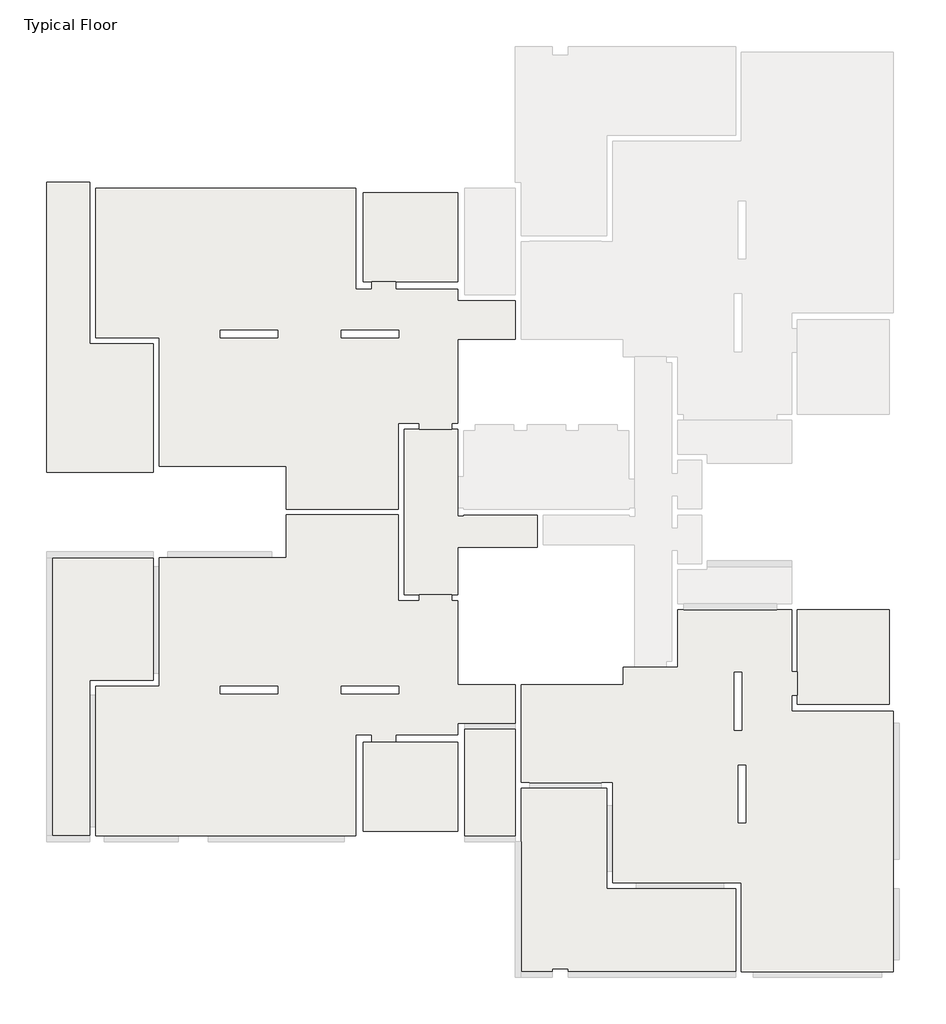
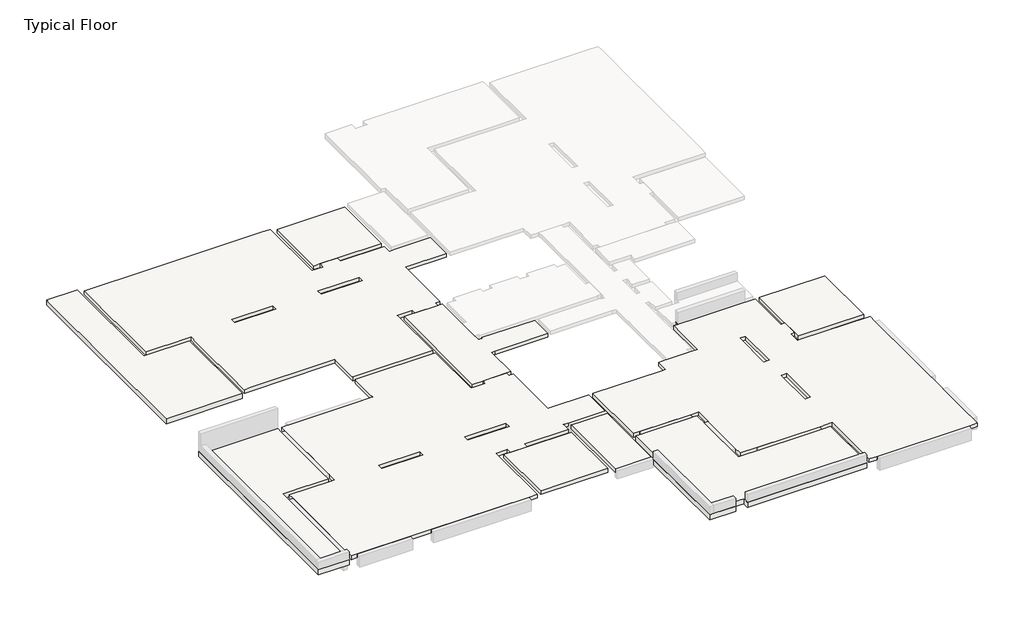
# One storey, part 1 of 2: 11 slabs.
"""IFC4 building model written with IfcOpenShell, lengths in millimetres."""

from ifc_helpers import new_model, si_unit, frame, origin, place, context, project, spatial, polyline, outline, extrude, faceted_brep, element, save

model = new_model("IFC4")

# Units and contexts
model_context = context("Model", 3, world=origin())
ifc_project = project(units=[si_unit("LENGTHUNIT", "METRE", prefix="MILLI")], contexts=[model_context])

# Site, building, storey
site = spatial("IfcSite", under=ifc_project)
building = spatial("IfcBuilding", under=site)
storey = spatial("IfcBuildingStorey", under=building, Name="Typical Floor", Elevation=3000.0)

# Slabs
placement = place(None, origin())
element("IfcSlab", 1, ObjectType="18", at=placement, inside=storey, context=model_context, shape_type="Brep", body=[
    faceted_brep([(-3147.0483227, 11035.7061689, 2820.0), (-2602.0483227, 11035.7061689, 2820.0), (-2602.0483227, 11285.7061689, 2820.0), (-1797.0483227, 11285.7061689, 2820.0), (-1797.0483227, 11035.7061689, 2820.0), (292.9516773, 11035.7061689, 2820.0), (292.9516773, 10641.3507002, 2820.0), (2246.4257984, 10641.3507002, 2820.0), (2246.4257984, 9337.0757978, 2820.0), (306.4257984, 9337.0757978, 2820.0), (306.4257984, 9137.0757978, 2820.0), (306.4257984, 6491.5264814, 2820.0), (96.4257984, 6491.5264814, 2820.0), (96.4257984, 6291.5264814, 2820.0), (-1004.8486157, 6291.5264814, 2820.0), (-1004.8486157, 6491.5264814, 2820.0), (-1704.8486157, 6491.5264814, 2820.0), (-1704.8486157, 6291.5264814, 2820.0), (-1704.8486157, 3590.0103681, 2820.0), (-5499.4457837, 3590.0103681, 2820.0), (-5499.4457837, 3661.3116377, 2820.0), (-5499.4457837, 4839.8443525, 2820.0), (-5499.4457837, 5039.8443525, 2820.0), (-5999.4457837, 5039.8443525, 2820.0), (-9505.5395337, 5039.8443525, 2820.0), (-9805.5395337, 5039.8443525, 2820.0), (-9805.5395337, 5339.8443525, 2820.0), (-9805.5395337, 8939.7491377, 2820.0), (-9805.5395337, 9386.8536298, 2820.0), (-10005.5395337, 9386.8536298, 2820.0), (-11954.2455884, 9386.8536298, 2820.0), (-11954.2455884, 14141.4166181, 2820.0), (-11954.2455884, 14441.4166181, 2820.0), (-11654.2455884, 14441.4166181, 2820.0), (-3147.0483227, 14441.4166181, 2820.0), (-3147.0483227, 11285.7061689, 2820.0), (-5784.0917798, 9641.1944502, 2820.0), (-7730.9496899, 9641.1944502, 2820.0), (-7730.9496899, 9391.1944502, 2820.0), (-5784.0917798, 9391.1944502, 2820.0), (-1703.720686, 9641.1944502, 2820.0), (-3648.408186, 9641.1944502, 2820.0), (-3648.408186, 9391.1944502, 2820.0), (-1703.720686, 9391.1944502, 2820.0), (-2602.0483227, 11035.7061689, 3000.0), (-3147.0483227, 11035.7061689, 3000.0), (-3147.0483227, 11285.7061689, 3000.0), (-3147.0483227, 14441.4166181, 3000.0), (-3547.0483227, 14441.4166181, 3000.0), (-8149.7387524, 14441.4166181, 3000.0), (-9154.7387524, 14441.4166181, 3000.0), (-11654.2455884, 14441.4166181, 3000.0), (-11954.2455884, 14441.4166181, 3000.0), (-11954.2455884, 14141.4166181, 3000.0), (-11954.2455884, 9686.3702314, 3000.0), (-11954.2455884, 9386.8536298, 3000.0), (-10005.5395337, 9386.8536298, 3000.0), (-9805.5395337, 9386.8536298, 3000.0), (-9805.5395337, 8939.7491377, 3000.0), (-9805.5395337, 5339.8443525, 3000.0), (-9805.5395337, 5039.8443525, 3000.0), (-9505.5395337, 5039.8443525, 3000.0), (-5999.4457837, 5039.8443525, 3000.0), (-5499.4457837, 5039.8443525, 3000.0), (-5499.4457837, 4839.8443525, 3000.0), (-5499.4457837, 3661.3116377, 3000.0), (-5499.4457837, 3590.0103681, 3000.0), (-5004.9145337, 3590.0103681, 3000.0), (-1704.8486157, 3590.0103681, 3000.0), (-1704.8486157, 6291.5264814, 3000.0), (-1704.8486157, 6491.5264814, 3000.0), (-1004.8486157, 6491.5264814, 3000.0), (-1004.8486157, 6291.5264814, 3000.0), (96.4257984, 6291.5264814, 3000.0), (96.4257984, 6491.5264814, 3000.0), (306.4257984, 6491.5264814, 3000.0), (306.4257984, 9137.0757978, 3000.0), (306.4257984, 9337.0757978, 3000.0), (2246.4257984, 9337.0757978, 3000.0), (2246.4257984, 10641.3507002, 3000.0), (542.9516773, 10641.3507002, 3000.0), (292.9516773, 10641.3507002, 3000.0), (292.9516773, 11035.7061689, 3000.0), (-1797.0483227, 11035.7061689, 3000.0), (-1797.0483227, 11285.7061689, 3000.0), (-2602.0483227, 11285.7061689, 3000.0), (-7730.9496899, 9641.1944502, 3000.0), (-5784.0917798, 9641.1944502, 3000.0), (-5784.0917798, 9391.1944502, 3000.0), (-7730.9496899, 9391.1944502, 3000.0), (-3648.408186, 9641.1944502, 3000.0), (-1703.720686, 9641.1944502, 3000.0), (-1703.720686, 9391.1944502, 3000.0), (-3648.408186, 9391.1944502, 3000.0)], [[[0, 1, 2, 3, 4, 5, 6, 7, 8, 9, 10, 11, 12, 13, 14, 15, 16, 17, 18, 19, 20, 21, 22, 23, 24, 25, 26, 27, 28, 29, 30, 31, 32, 33, 34, 35], [36, 37, 38, 39], [40, 41, 42, 43]], [[44, 45, 46, 47, 48, 49, 50, 51, 52, 53, 54, 55, 56, 57, 58, 59, 60, 61, 62, 63, 64, 65, 66, 67, 68, 69, 70, 71, 72, 73, 74, 75, 76, 77, 78, 79, 80, 81, 82, 83, 84, 85], [86, 87, 88, 89], [90, 91, 92, 93]], [[45, 0, 35, 34, 47, 46]], [[1, 0, 45, 44]], [[2, 1, 44, 85]], [[3, 2, 85, 84]], [[4, 3, 84, 83]], [[4, 83, 82, 5]], [[79, 7, 6, 81, 80]], [[8, 7, 79, 78]], [[9, 8, 78, 77]], [[9, 77, 76, 75, 11, 10]], [[12, 11, 75, 74]], [[13, 12, 74, 73]], [[14, 13, 73, 72]], [[15, 14, 72, 71]], [[16, 15, 71, 70]], [[16, 70, 69, 68, 18, 17]], [[19, 18, 68, 67, 66]], [[19, 66, 65, 64, 63, 22, 21, 20]], [[22, 63, 62, 61, 60, 25, 24, 23]], [[25, 60, 59, 58, 57, 28, 27, 26]], [[28, 57, 56, 55, 30, 29]], [[30, 55, 54, 53, 52, 32, 31]], [[32, 52, 51, 50, 49, 48, 47, 34, 33]], [[37, 36, 87, 86]], [[38, 37, 86, 89]], [[39, 38, 89, 88]], [[36, 39, 88, 87]], [[41, 40, 91, 90]], [[42, 41, 90, 93]], [[43, 42, 93, 92]], [[40, 43, 92, 91]], [[81, 6, 5, 82]]]),
])
element("IfcSlab", 2, ObjectType="18", at=placement, inside=storey, context=model_context, shape_type="Brep", body=[
    faceted_brep([(292.9516773, 14291.4166181, 2820.0), (292.9516773, 11285.7061689, 2820.0), (-1797.0483227, 11285.7061689, 2820.0), (-2602.0483227, 11285.7061689, 2820.0), (-2897.0483227, 11285.7061689, 2820.0), (-2897.0483227, 14291.4166181, 2820.0), (292.9516773, 11285.7061689, 3000.0), (292.9516773, 14291.4166181, 3000.0), (-2897.0483227, 14291.4166181, 3000.0), (-2897.0483227, 11285.7061689, 3000.0), (-2602.0483227, 11285.7061689, 3000.0), (-1797.0483227, 11285.7061689, 3000.0)], [[[0, 1, 2, 3, 4, 5]], [[6, 7, 8, 9, 10, 11]], [[1, 0, 7, 6]], [[1, 6, 11, 10, 9, 4, 3, 2]], [[5, 4, 9, 8]], [[0, 5, 8, 7]]]),
])
element("IfcSlab", 3, ObjectType="18", at=placement, inside=storey, context=model_context, shape_type="Brep", body=[
    faceted_brep([(-2602.0483227, -4055.6854327, 2820.0), (-3147.0483227, -4055.6854327, 2820.0), (-3147.0483227, -4305.6854327, 2820.0), (-3147.0483227, -7461.3958819, 2820.0), (-3547.0483227, -7461.3958819, 2820.0), (-3547.0483227, -7466.3958819, 2820.0), (-8149.7387524, -7466.3958819, 2820.0), (-8149.7387524, -7461.3958819, 2820.0), (-9154.7387524, -7461.3958819, 2820.0), (-9154.7387524, -7466.3958819, 2820.0), (-11654.2455884, -7466.3958819, 2820.0), (-11654.2455884, -7461.3958819, 2820.0), (-11954.2455884, -7461.3958819, 2820.0), (-11954.2455884, -7161.3958819, 2820.0), (-11954.2455884, -2406.8328936, 2820.0), (-10005.5395337, -2406.8328936, 2820.0), (-9805.5395337, -2406.8328936, 2820.0), (-9805.5395337, -1959.7284014, 2820.0), (-9805.5395337, 1640.1763837, 2820.0), (-9805.5395337, 1940.1763837, 2820.0), (-9505.5395337, 1940.1763837, 2820.0), (-5999.4457837, 1940.1763837, 2820.0), (-5499.4457837, 1940.1763837, 2820.0), (-5499.4457837, 2140.1763837, 2820.0), (-5499.4457837, 3320.5572431, 2820.0), (-5499.4457837, 3390.0103681, 2820.0), (-1704.8486157, 3390.0103681, 2820.0), (-1704.8486157, 491.1895673, 2820.0), (-999.8486157, 491.1895673, 2820.0), (-999.8486157, 688.4942548, 2820.0), (96.4257984, 688.4942548, 2820.0), (96.4257984, 488.4942548, 2820.0), (306.4257984, 488.4942548, 2820.0), (306.4257984, -2157.0550616, 2820.0), (306.4257984, -2357.0550616, 2820.0), (2246.4257984, -2357.0550616, 2820.0), (2246.4257984, -3661.3299639, 2820.0), (292.9516773, -3661.3299639, 2820.0), (292.9516773, -4055.6854327, 2820.0), (-1797.0483227, -4055.6854327, 2820.0), (-1797.0483227, -4305.6854327, 2820.0), (-2602.0483227, -4305.6854327, 2820.0), (-7730.9496899, -2661.1737139, 2820.0), (-5784.0917798, -2661.1737139, 2820.0), (-5784.0917798, -2411.1737139, 2820.0), (-7730.9496899, -2411.1737139, 2820.0), (-3648.408186, -2661.1737139, 2820.0), (-1703.720686, -2661.1737139, 2820.0), (-1703.720686, -2411.1737139, 2820.0), (-3648.408186, -2411.1737139, 2820.0), (-3147.0483227, -4055.6854327, 3000.0), (-2602.0483227, -4055.6854327, 3000.0), (-2602.0483227, -4305.6854327, 3000.0), (-1797.0483227, -4305.6854327, 3000.0), (-1797.0483227, -4055.6854327, 3000.0), (292.9516773, -4055.6854327, 3000.0), (292.9516773, -3661.3299639, 3000.0), (542.9516773, -3661.3299639, 3000.0), (2246.4257984, -3661.3299639, 3000.0), (2246.4257984, -2357.0550616, 3000.0), (306.4257984, -2357.0550616, 3000.0), (306.4257984, -2157.0550616, 3000.0), (306.4257984, 488.4942548, 3000.0), (96.4257984, 488.4942548, 3000.0), (96.4257984, 688.4942548, 3000.0), (-999.8486157, 688.4942548, 3000.0), (-999.8486157, 491.1895673, 3000.0), (-1504.8486157, 491.1895673, 3000.0), (-1704.8486157, 491.1895673, 3000.0), (-1704.8486157, 3390.0103681, 3000.0), (-5004.9145337, 3390.0103681, 3000.0), (-5499.4457837, 3390.0103681, 3000.0), (-5499.4457837, 3320.5572431, 3000.0), (-5499.4457837, 2140.1763837, 3000.0), (-5499.4457837, 1940.1763837, 3000.0), (-5999.4457837, 1940.1763837, 3000.0), (-9505.5395337, 1940.1763837, 3000.0), (-9805.5395337, 1940.1763837, 3000.0), (-9805.5395337, 1640.1763837, 3000.0), (-9805.5395337, -1959.7284014, 3000.0), (-9805.5395337, -2406.8328936, 3000.0), (-10005.5395337, -2406.8328936, 3000.0), (-11954.2455884, -2406.8328936, 3000.0), (-11954.2455884, -2706.3494952, 3000.0), (-11954.2455884, -7161.3958819, 3000.0), (-11954.2455884, -7461.3958819, 3000.0), (-11654.2455884, -7461.3958819, 3000.0), (-11654.2455884, -7466.3958819, 3000.0), (-9154.7387524, -7466.3958819, 3000.0), (-9154.7387524, -7461.3958819, 3000.0), (-8149.7387524, -7461.3958819, 3000.0), (-8149.7387524, -7466.3958819, 3000.0), (-3547.0483227, -7466.3958819, 3000.0), (-3547.0483227, -7461.3958819, 3000.0), (-3147.0483227, -7461.3958819, 3000.0), (-3147.0483227, -4305.6854327, 3000.0), (-5784.0917798, -2661.1737139, 3000.0), (-7730.9496899, -2661.1737139, 3000.0), (-7730.9496899, -2411.1737139, 3000.0), (-5784.0917798, -2411.1737139, 3000.0), (-1703.720686, -2661.1737139, 3000.0), (-3648.408186, -2661.1737139, 3000.0), (-3648.408186, -2411.1737139, 3000.0), (-1703.720686, -2411.1737139, 3000.0)], [[[0, 1, 2, 3, 4, 5, 6, 7, 8, 9, 10, 11, 12, 13, 14, 15, 16, 17, 18, 19, 20, 21, 22, 23, 24, 25, 26, 27, 28, 29, 30, 31, 32, 33, 34, 35, 36, 37, 38, 39, 40, 41], [42, 43, 44, 45], [46, 47, 48, 49]], [[50, 51, 52, 53, 54, 55, 56, 57, 58, 59, 60, 61, 62, 63, 64, 65, 66, 67, 68, 69, 70, 71, 72, 73, 74, 75, 76, 77, 78, 79, 80, 81, 82, 83, 84, 85, 86, 87, 88, 89, 90, 91, 92, 93, 94, 95], [96, 97, 98, 99], [100, 101, 102, 103]], [[1, 50, 95, 94, 3, 2]], [[1, 0, 51, 50]], [[0, 41, 52, 51]], [[41, 40, 53, 52]], [[40, 39, 54, 53]], [[54, 39, 38, 55]], [[36, 58, 57, 56, 37]], [[36, 35, 59, 58]], [[35, 34, 60, 59]], [[32, 62, 61, 60, 34, 33]], [[32, 31, 63, 62]], [[31, 30, 64, 63]], [[64, 30, 29, 65]], [[26, 69, 68, 27]], [[26, 25, 71, 70, 69]], [[22, 74, 73, 72, 71, 25, 24, 23]], [[19, 77, 76, 75, 74, 22, 21, 20]], [[16, 80, 79, 78, 77, 19, 18, 17]], [[14, 82, 81, 80, 16, 15]], [[82, 14, 13, 12, 85, 84, 83]], [[87, 10, 9, 88]], [[91, 6, 5, 92]], [[43, 42, 97, 96]], [[42, 45, 98, 97]], [[45, 44, 99, 98]], [[44, 43, 96, 99]], [[47, 46, 101, 100]], [[46, 49, 102, 101]], [[49, 48, 103, 102]], [[48, 47, 100, 103]], [[86, 11, 10, 87]], [[11, 86, 85, 12]], [[27, 68, 67, 66, 28]], [[28, 66, 65, 29]], [[37, 56, 55, 38]], [[7, 90, 89, 8]], [[90, 7, 6, 91]], [[8, 89, 88, 9]], [[93, 4, 3, 94]], [[4, 93, 92, 5]]]),
])
element("IfcSlab", 4, ObjectType="18", at=placement, inside=storey, context=model_context, shape_type="Brep", body=[
    faceted_brep([(292.9516773, -4305.6854327, 2820.0), (292.9516773, -7311.3958819, 2820.0), (-2897.0483227, -7311.3958819, 2820.0), (-2897.0483227, -4305.6854327, 2820.0), (-2602.0483227, -4305.6854327, 2820.0), (-1797.0483227, -4305.6854327, 2820.0), (292.9516773, -7311.3958819, 3000.0), (292.9516773, -4305.6854327, 3000.0), (-1797.0483227, -4305.6854327, 3000.0), (-2602.0483227, -4305.6854327, 3000.0), (-2897.0483227, -4305.6854327, 3000.0), (-2897.0483227, -7311.3958819, 3000.0)], [[[0, 1, 2, 3, 4, 5]], [[6, 7, 8, 9, 10, 11]], [[1, 0, 7, 6]], [[3, 10, 9, 8, 7, 0, 5, 4]], [[3, 2, 11, 10]], [[2, 1, 6, 11]]]),
])
element("IfcSlab", 5, ObjectType="18", at=placement, inside=storey, context=model_context, shape_type="SweptSolid", body=[
    extrude(outline(polyline([(2246.4257984, -3861.3299639), (2246.4257984, -7461.3958819), (542.9516773, -7461.3958819), (542.9516773, -3861.3299639), (2246.4257984, -3861.3299639)])), frame((0.0, 0.0, 2820.0), z_axis=(0.0, 0.0, 1.0), x_axis=(1.0, 0.0, 0.0)), (0.0, 0.0, 1.0), 180.0),
])
element("IfcSlab", 6, ObjectType="18", at=placement, inside=storey, context=model_context, shape_type="Brep", body=[
    faceted_brep([(11796.5527515, -2710.0457842, 2820.0), (11596.5527515, -2710.0457842, 2820.0), (11596.5527515, -3259.804085, 2820.0), (15047.1826343, -3259.804085, 2820.0), (15047.1826343, -12061.3104327, 2820.0), (14652.4902515, -12061.3104327, 2820.0), (14652.4902515, -12066.3104327, 2820.0), (10302.4292163, -12066.3104327, 2820.0), (10302.4292163, -12061.3104327, 2820.0), (9902.4292163, -12061.3104327, 2820.0), (9902.4292163, -9261.9354327, 2820.0), (9902.4292163, -9061.9354327, 2820.0), (9302.4292163, -9061.9354327, 2820.0), (6350.1123218, -9061.9354327, 2820.0), (5545.4492359, -9061.9354327, 2820.0), (5545.4492359, -8661.9549639, 2820.0), (5545.4492359, -6456.8182452, 2820.0), (5545.4492359, -5860.2777178, 2820.0), (5545.4492359, -5660.2777178, 2820.0), (5152.6049976, -5660.2777178, 2820.0), (5152.6049976, -5665.2777178, 2820.0), (2745.6201343, -5665.2777178, 2820.0), (2745.6201343, -5660.2777178, 2820.0), (2446.4257984, -5660.2777178, 2820.0), (2446.4257984, -2357.0550616, 2820.0), (5901.4257984, -2357.0550616, 2820.0), (5901.4257984, -1759.7284014, 2820.0), (6296.4111499, -1759.7284014, 2820.0), (7351.2304859, -1759.7284014, 2820.0), (7351.2304859, -1760.3729327, 2820.0), (7751.2304859, -1760.3729327, 2820.0), (7751.2304859, -1560.3729327, 2820.0), (7751.2304859, 188.6553877, 2820.0), (7955.5859546, 188.6553877, 2820.0), (7955.5859546, 388.6553877, 2820.0), (11103.869646, 388.6553877, 2820.0), (11103.869646, 188.6553877, 2820.0), (11596.5527515, 188.6553877, 2820.0), (11596.5527515, -1909.8089678, 2820.0), (11796.5527515, -1909.8089678, 2820.0), (10046.8798999, -7025.4657061, 2820.0), (10046.8798999, -5082.9486163, 2820.0), (9796.8798999, -5082.9486163, 2820.0), (9796.8798999, -7025.4657061, 2820.0), (9906.2060718, -3891.3934405, 2820.0), (9906.2060718, -1940.19471, 2820.0), (9656.2060718, -1940.19471, 2820.0), (9656.2060718, -3891.3934405, 2820.0), (11596.5527515, -2710.0457842, 3000.0), (11796.5527515, -2710.0457842, 3000.0), (11796.5527515, -1909.8089678, 3000.0), (11596.5527515, -1909.8089678, 3000.0), (11596.5527515, 188.6553877, 3000.0), (11103.869646, 188.6553877, 3000.0), (11103.869646, 388.6553877, 3000.0), (7955.5859546, 388.6553877, 3000.0), (7955.5859546, 188.6553877, 3000.0), (7751.2304859, 188.6553877, 3000.0), (7751.2304859, -1560.3729327, 3000.0), (7751.2304859, -1760.3729327, 3000.0), (7351.2304859, -1760.3729327, 3000.0), (7351.2304859, -1759.7284014, 3000.0), (6296.4111499, -1759.7284014, 3000.0), (5901.4257984, -1759.7284014, 3000.0), (5901.4257984, -2357.0550616, 3000.0), (5701.4257984, -2357.0550616, 3000.0), (2446.4257984, -2357.0550616, 3000.0), (2446.4257984, -5660.2777178, 3000.0), (2745.6201343, -5660.2777178, 3000.0), (2745.6201343, -5665.2777178, 3000.0), (5152.6049976, -5665.2777178, 3000.0), (5152.6049976, -5660.2777178, 3000.0), (5545.4492359, -5660.2777178, 3000.0), (5545.4492359, -5860.2777178, 3000.0), (5545.4492359, -6456.8182452, 3000.0), (5545.4492359, -8661.9549639, 3000.0), (5545.4492359, -9061.9354327, 3000.0), (6350.1123218, -9061.9354327, 3000.0), (9302.4292163, -9061.9354327, 3000.0), (9902.4292163, -9061.9354327, 3000.0), (9902.4292163, -9261.9354327, 3000.0), (9902.4292163, -12061.3104327, 3000.0), (10302.4292163, -12061.3104327, 3000.0), (10302.4292163, -12066.3104327, 3000.0), (14652.4902515, -12066.3104327, 3000.0), (14652.4902515, -12061.3104327, 3000.0), (15047.1826343, -12061.3104327, 3000.0), (15047.1826343, -11661.3104327, 3000.0), (15047.1826343, -9252.3065264, 3000.0), (15047.1826343, -8260.429085, 3000.0), (15047.1826343, -3654.8187334, 3000.0), (15047.1826343, -3259.804085, 3000.0), (11796.5527515, -3259.804085, 3000.0), (11596.5527515, -3259.804085, 3000.0), (11596.5527515, -2710.6903155, 3000.0), (10046.8798999, -5082.9486163, 3000.0), (10046.8798999, -7025.4657061, 3000.0), (9796.8798999, -7025.4657061, 3000.0), (9796.8798999, -5082.9486163, 3000.0), (9906.2060718, -1940.19471, 3000.0), (9906.2060718, -3891.3934405, 3000.0), (9656.2060718, -3891.3934405, 3000.0), (9656.2060718, -1940.19471, 3000.0)], [[[0, 1, 2, 3, 4, 5, 6, 7, 8, 9, 10, 11, 12, 13, 14, 15, 16, 17, 18, 19, 20, 21, 22, 23, 24, 25, 26, 27, 28, 29, 30, 31, 32, 33, 34, 35, 36, 37, 38, 39], [40, 41, 42, 43], [44, 45, 46, 47]], [[48, 49, 50, 51, 52, 53, 54, 55, 56, 57, 58, 59, 60, 61, 62, 63, 64, 65, 66, 67, 68, 69, 70, 71, 72, 73, 74, 75, 76, 77, 78, 79, 80, 81, 82, 83, 84, 85, 86, 87, 88, 89, 90, 91, 92, 93, 94], [95, 96, 97, 98], [99, 100, 101, 102]], [[69, 21, 20, 70]], [[14, 76, 75, 74, 73, 72, 18, 17, 16, 15]], [[11, 79, 78, 77, 76, 14, 13, 12]], [[79, 11, 10, 9, 81, 80]], [[83, 7, 6, 84]], [[3, 91, 90, 89, 88, 87, 86, 4]], [[1, 48, 94, 93, 2]], [[1, 0, 49, 48]], [[49, 0, 39, 50]], [[51, 38, 37, 52]], [[30, 59, 58, 57, 32, 31]], [[26, 63, 62, 61, 28, 27]], [[63, 26, 25, 64]], [[66, 24, 23, 67]], [[22, 68, 67, 23]], [[68, 22, 21, 69]], [[18, 72, 71, 19]], [[19, 71, 70, 20]], [[40, 96, 95, 41]], [[42, 98, 97, 43]], [[41, 95, 98, 42]], [[96, 40, 43, 97]], [[44, 100, 99, 45]], [[46, 102, 101, 47]], [[45, 99, 102, 46]], [[100, 44, 47, 101]], [[91, 3, 2, 93, 92]], [[38, 51, 50, 39]], [[36, 53, 52, 37]], [[29, 60, 59, 30]], [[60, 29, 28, 61]], [[56, 33, 32, 57]], [[33, 56, 55, 34]], [[35, 34, 55, 54]], [[53, 36, 35, 54]], [[64, 25, 24, 66, 65]], [[8, 82, 81, 9]], [[82, 8, 7, 83]], [[85, 5, 4, 86]], [[5, 85, 84, 6]]]),
])
element("IfcSlab", 7, ObjectType="18", at=placement, inside=storey, context=model_context, shape_type="Brep", body=[
    faceted_brep([(14897.1826343, 188.5748212, 2820.0), (14897.1826343, -3009.804085, 2820.0), (11796.5527515, -3009.804085, 2820.0), (11796.5527515, -2710.0457842, 2820.0), (11796.5527515, -1909.8089678, 2820.0), (11796.5527515, -1909.1644366, 2820.0), (11796.5527515, 188.5748212, 2820.0), (14897.1826343, -3009.804085, 3000.0), (14897.1826343, 188.5748212, 3000.0), (11796.5527515, 188.5748212, 3000.0), (11796.5527515, -1909.1644366, 3000.0), (11796.5527515, -1909.8089678, 3000.0), (11796.5527515, -2710.0457842, 3000.0), (11796.5527515, -2710.6903155, 3000.0), (11796.5527515, -3009.804085, 3000.0)], [[[0, 1, 2, 3, 4, 5, 6]], [[7, 8, 9, 10, 11, 12, 13, 14]], [[1, 0, 8, 7]], [[0, 6, 9, 8]], [[2, 14, 13, 12, 11, 10, 9, 6, 5, 4, 3]], [[2, 1, 7, 14]]]),
])
element("IfcSlab", 8, ObjectType="18", at=placement, inside=storey, context=model_context, shape_type="Brep", body=[
    faceted_brep([(306.4257984, 6291.5264814, 2820.0), (306.4257984, 4687.0757978, 2820.0), (306.4257984, 3635.0909345, 2820.0), (301.7382984, 3635.0909345, 2820.0), (301.7382984, 3340.0909345, 2820.0), (501.7382984, 3340.0909345, 2820.0), (501.7382984, 3385.0909345, 2820.0), (2997.0654468, 3385.0909345, 2820.0), (2997.0654468, 2292.9449384, 2820.0), (506.4257984, 2292.9449384, 2820.0), (306.4257984, 2292.9449384, 2820.0), (306.4257984, 688.4942548, 2820.0), (96.4257984, 688.4942548, 2820.0), (-999.8486157, 688.4942548, 2820.0), (-999.8486157, 691.1895673, 2820.0), (-1504.8486157, 691.1895673, 2820.0), (-1504.8486157, 6291.5264814, 2820.0), (-1004.8486157, 6291.5264814, 2820.0), (96.4257984, 6291.5264814, 2820.0), (306.4257984, 4687.0757978, 3000.0), (306.4257984, 6291.5264814, 3000.0), (96.4257984, 6291.5264814, 3000.0), (-1004.8486157, 6291.5264814, 3000.0), (-1504.8486157, 6291.5264814, 3000.0), (-1504.8486157, 691.1895673, 3000.0), (-999.8486157, 691.1895673, 3000.0), (-999.8486157, 688.4942548, 3000.0), (96.4257984, 688.4942548, 3000.0), (306.4257984, 688.4942548, 3000.0), (306.4257984, 2292.9449384, 3000.0), (506.4257984, 2292.9449384, 3000.0), (2997.0654468, 2292.9449384, 3000.0), (2997.0654468, 3385.0909345, 3000.0), (501.7382984, 3385.0909345, 3000.0), (501.7382984, 3340.0909345, 3000.0), (301.7382984, 3340.0909345, 3000.0), (301.7382984, 3635.0909345, 3000.0), (306.4257984, 3635.0909345, 3000.0)], [[[0, 1, 2, 3, 4, 5, 6, 7, 8, 9, 10, 11, 12, 13, 14, 15, 16, 17, 18]], [[19, 20, 21, 22, 23, 24, 25, 26, 27, 28, 29, 30, 31, 32, 33, 34, 35, 36, 37]], [[1, 0, 20, 19]], [[2, 1, 19, 37]], [[3, 2, 37, 36]], [[4, 3, 36, 35]], [[5, 4, 35, 34]], [[6, 5, 34, 33]], [[7, 6, 33, 32]], [[8, 7, 32, 31]], [[9, 8, 31, 30]], [[10, 9, 30, 29]], [[11, 10, 29, 28]], [[11, 28, 27, 26, 13, 12]], [[14, 13, 26, 25]], [[15, 14, 25, 24]], [[16, 15, 24, 23]], [[16, 23, 22, 21, 20, 0, 18, 17]]]),
])
element("IfcSlab", 9, ObjectType="25", at=placement, inside=storey, context=model_context, shape_type="Brep", body=[
    faceted_brep([(-10005.5395337, 4839.8443525, 2750.0), (-13614.2455884, 4839.8443525, 2750.0), (-13614.2455884, 14641.4166181, 2750.0), (-12154.2455884, 14641.4166181, 2750.0), (-12154.2455884, 14141.4166181, 2750.0), (-12154.2455884, 9686.3702314, 2750.0), (-12154.2455884, 9186.8536298, 2750.0), (-11954.2455884, 9186.8536298, 2750.0), (-10005.5395337, 9186.8536298, 2750.0), (-13614.2455884, 4839.8443525, 3000.0), (-13414.2455884, 4839.8443525, 3000.0), (-10005.5395337, 4839.8443525, 3000.0), (-10005.5395337, 5039.8443525, 3000.0), (-10005.5395337, 5339.8443525, 3000.0), (-10005.5395337, 8939.7491377, 3000.0), (-10005.5395337, 9186.8536298, 3000.0), (-11954.2455884, 9186.8536298, 3000.0), (-12154.2455884, 9186.8536298, 3000.0), (-12154.2455884, 9686.3702314, 3000.0), (-12154.2455884, 14141.4166181, 3000.0), (-12154.2455884, 14441.4166181, 3000.0), (-12154.2455884, 14641.4166181, 3000.0), (-13614.2455884, 14641.4166181, 3000.0), (-13614.2455884, 14441.4166181, 3000.0)], [[[0, 1, 2, 3, 4, 5, 6, 7, 8]], [[9, 10, 11, 12, 13, 14, 15, 16, 17, 18, 19, 20, 21, 22, 23]], [[1, 0, 11, 10, 9]], [[2, 1, 9, 23, 22]], [[3, 2, 22, 21]], [[3, 21, 20, 19, 18, 17, 6, 5, 4]], [[6, 17, 16, 15, 8, 7]], [[0, 8, 15, 14, 13, 12, 11]]]),
])
element("IfcSlab", 10, ObjectType="25", at=placement, inside=storey, context=model_context, shape_type="Brep", body=[
    faceted_brep([(-13614.2455884, 2140.1763837, 2750.0), (-10005.5395337, 2140.1763837, 2750.0), (-10005.5395337, -2206.8328936, 2750.0), (-11954.2455884, -2206.8328936, 2750.0), (-12154.2455884, -2206.8328936, 2750.0), (-12154.2455884, -2706.3494952, 2750.0), (-12154.2455884, -7161.3958819, 2750.0), (-12154.2455884, -7661.3958819, 2750.0), (-13614.2455884, -7661.3958819, 2750.0), (-10005.5395337, 2140.1763837, 3000.0), (-13414.2455884, 2140.1763837, 3000.0), (-13614.2455884, 2140.1763837, 3000.0), (-13614.2455884, -7461.3958819, 3000.0), (-13614.2455884, -7661.3958819, 3000.0), (-12154.2455884, -7661.3958819, 3000.0), (-12154.2455884, -7461.3958819, 3000.0), (-12154.2455884, -7161.3958819, 3000.0), (-12154.2455884, -2706.3494952, 3000.0), (-12154.2455884, -2206.8328936, 3000.0), (-11954.2455884, -2206.8328936, 3000.0), (-10005.5395337, -2206.8328936, 3000.0), (-10005.5395337, -1959.7284014, 3000.0), (-10005.5395337, 1640.1763837, 3000.0), (-10005.5395337, 1940.1763837, 3000.0)], [[[0, 1, 2, 3, 4, 5, 6, 7, 8]], [[9, 10, 11, 12, 13, 14, 15, 16, 17, 18, 19, 20, 21, 22, 23]], [[1, 0, 11, 10, 9]], [[0, 8, 13, 12, 11]], [[8, 7, 14, 13]], [[4, 18, 17, 16, 15, 14, 7, 6, 5]], [[2, 20, 19, 18, 4, 3]], [[2, 1, 9, 23, 22, 21, 20]]]),
])
element("IfcSlab", 11, ObjectType="25", at=placement, inside=storey, context=model_context, shape_type="Brep", body=[
    faceted_brep([(3495.6958179, -12260.9784014, 2750.0), (2246.4257984, -12260.9784014, 2750.0), (2246.4257984, -7661.3958819, 2750.0), (2446.4257984, -7661.3958819, 2750.0), (2446.4257984, -5860.2777178, 2750.0), (5345.4492359, -5860.2777178, 2750.0), (5345.4492359, -6456.8182452, 2750.0), (5345.4492359, -8661.9549639, 2750.0), (5345.4492359, -9261.9354327, 2750.0), (5545.4492359, -9261.9354327, 2750.0), (6350.1123218, -9261.9354327, 2750.0), (9302.4292163, -9261.9354327, 2750.0), (9702.4292163, -9261.9354327, 2750.0), (9702.4292163, -12261.3104327, 2750.0), (4045.6958179, -12261.3104327, 2750.0), (4045.6958179, -12260.9784014, 2750.0), (4045.6958179, -11960.9784014, 2750.0), (3495.6958179, -11960.9784014, 2750.0), (2246.4257984, -12260.9784014, 3000.0), (2446.4257984, -12260.9784014, 3000.0), (3495.6958179, -12260.9784014, 3000.0), (3495.6958179, -12060.9784014, 3000.0), (3495.6958179, -11960.9784014, 3000.0), (4045.6958179, -11960.9784014, 3000.0), (4045.6958179, -12061.3104327, 3000.0), (4045.6958179, -12260.9784014, 3000.0), (4045.6958179, -12261.3104327, 3000.0), (9702.4292163, -12261.3104327, 3000.0), (9702.4292163, -12061.3104327, 3000.0), (9702.4292163, -9261.9354327, 3000.0), (9302.4292163, -9261.9354327, 3000.0), (6350.1123218, -9261.9354327, 3000.0), (5545.4492359, -9261.9354327, 3000.0), (5345.4492359, -9261.9354327, 3000.0), (5345.4492359, -8661.9549639, 3000.0), (5345.4492359, -6456.8182452, 3000.0), (5345.4492359, -5860.2777178, 3000.0), (5152.6049976, -5860.2777178, 3000.0), (2745.6201343, -5860.2777178, 3000.0), (2446.4257984, -5860.2777178, 3000.0), (2446.4257984, -7661.3958819, 3000.0), (2246.4257984, -7661.3958819, 3000.0)], [[[0, 1, 2, 3, 4, 5, 6, 7, 8, 9, 10, 11, 12, 13, 14, 15, 16, 17]], [[18, 19, 20, 21, 22, 23, 24, 25, 26, 27, 28, 29, 30, 31, 32, 33, 34, 35, 36, 37, 38, 39, 40, 41]], [[1, 0, 20, 19, 18]], [[0, 17, 22, 21, 20]], [[17, 16, 23, 22]], [[14, 26, 25, 24, 23, 16, 15]], [[14, 13, 27, 26]], [[13, 12, 29, 28, 27]], [[8, 33, 32, 31, 30, 29, 12, 11, 10, 9]], [[5, 36, 35, 34, 33, 8, 7, 6]], [[5, 4, 39, 38, 37, 36]], [[2, 1, 18, 41]], [[3, 2, 41, 40]], [[4, 3, 40, 39]]]),
])

save(model, "model.ifc")

# Revit data of these elements
# Type "18"
#   Function = 0
#   Layers, outside or top first: 18 cm "Concrete" (function 1)
# Type "25"
#   Function = 0
#   Layers, outside or top first: 25 cm "Concrete" (function 1)
# Element 1 (IfcSlab, "18")
#   Mark = "S5"
#   SOFiSTiK_AMG_Comments = ""
#   Height Offset From Level = 0 cm
#   built-in parameter 1001954 = 1
#   SOFiSTiK_AMG_Scheduled = yes
#   SOFiSTiK_AMG_Adjusted = yes
#   Phase Created = New Construction
#   Materials on its faces: "Concrete"
# Element 2 (IfcSlab, "18")
#   Mark = "S6"
#   SOFiSTiK_AMG_Comments = ""
#   Height Offset From Level = 0 cm
#   built-in parameter 1001954 = 1
#   SOFiSTiK_AMG_Scheduled = yes
#   SOFiSTiK_AMG_Adjusted = yes
#   Phase Created = New Construction
#   Materials on its faces: "Concrete"
# Element 3 (IfcSlab, "18")
#   Mark = "S10"
#   SOFiSTiK_AMG_Comments = ""
#   Height Offset From Level = 0 cm
#   built-in parameter 1001954 = 1
#   SOFiSTiK_AMG_Scheduled = yes
#   SOFiSTiK_AMG_Adjusted = yes
#   Phase Created = New Construction
#   Materials on its faces: "Concrete"
# Element 4 (IfcSlab, "18")
#   Mark = "S11"
#   SOFiSTiK_AMG_Comments = ""
#   Height Offset From Level = 0 cm
#   built-in parameter 1001954 = 1
#   SOFiSTiK_AMG_Scheduled = yes
#   SOFiSTiK_AMG_Adjusted = yes
#   Phase Created = New Construction
#   Materials on its faces: "Concrete"
# Element 5 (IfcSlab, "18")
#   Mark = "S12"
#   SOFiSTiK_AMG_Comments = ""
#   Height Offset From Level = 0 cm
#   built-in parameter 1001954 = 1
#   SOFiSTiK_AMG_Scheduled = yes
#   SOFiSTiK_AMG_Adjusted = yes
#   Phase Created = New Construction
#   Materials on its faces: "Concrete"
# Element 6 (IfcSlab, "18")
#   Mark = "S13"
#   SOFiSTiK_AMG_Comments = ""
#   built-in parameter 1001955 = -1.5708 (stored number, unit not read)
#   Height Offset From Level = 0 cm
#   built-in parameter 1001954 = 1
#   SOFiSTiK_AMG_Scheduled = yes
#   SOFiSTiK_AMG_Adjusted = yes
#   Phase Created = New Construction
#   Materials on its faces: "Concrete"
# Element 7 (IfcSlab, "18")
#   Mark = "S14"
#   SOFiSTiK_AMG_Comments = ""
#   Height Offset From Level = 0 cm
#   built-in parameter 1001954 = 1
#   SOFiSTiK_AMG_Scheduled = yes
#   SOFiSTiK_AMG_Adjusted = yes
#   Phase Created = New Construction
#   Materials on its faces: "Concrete"
# Element 8 (IfcSlab, "18")
#   Mark = "S18"
#   SOFiSTiK_AMG_Comments = ""
#   Height Offset From Level = 0 cm
#   built-in parameter 1001954 = 1
#   SOFiSTiK_AMG_Scheduled = yes
#   SOFiSTiK_AMG_Adjusted = no
#   Phase Created = New Construction
#   Materials on its faces: "Concrete"
# Element 9 (IfcSlab, "25")
#   Mark = "S1"
#   SOFiSTiK_AMG_Comments = ""
#   Height Offset From Level = 0 cm
#   built-in parameter 1001954 = 1
#   SOFiSTiK_AMG_Scheduled = yes
#   SOFiSTiK_AMG_Adjusted = yes
#   Phase Created = New Construction
#   Materials on its faces: "Concrete"
# Element 10 (IfcSlab, "25")
#   Mark = "S3"
#   SOFiSTiK_AMG_Comments = ""
#   Height Offset From Level = 0 cm
#   built-in parameter 1001954 = 1
#   SOFiSTiK_AMG_Scheduled = yes
#   SOFiSTiK_AMG_Adjusted = yes
#   Phase Created = New Construction
#   Materials on its faces: "Concrete"
# Element 11 (IfcSlab, "25")
#   Mark = "S4"
#   SOFiSTiK_AMG_Comments = ""
#   built-in parameter 1001955 = -1.5708 (stored number, unit not read)
#   Height Offset From Level = 0 cm
#   built-in parameter 1001954 = 1
#   SOFiSTiK_AMG_Scheduled = yes
#   SOFiSTiK_AMG_Adjusted = no
#   Phase Created = New Construction
#   Materials on its faces: "Concrete"
# Materials
#   "Concrete": class "Concrete", colour RGB 192 192 192, transparency 0, Keynote = "01000", Description = "Cast-in-place concrete", Cost = 0
